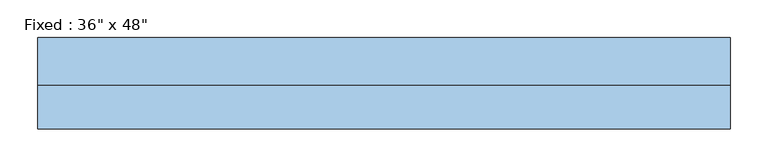
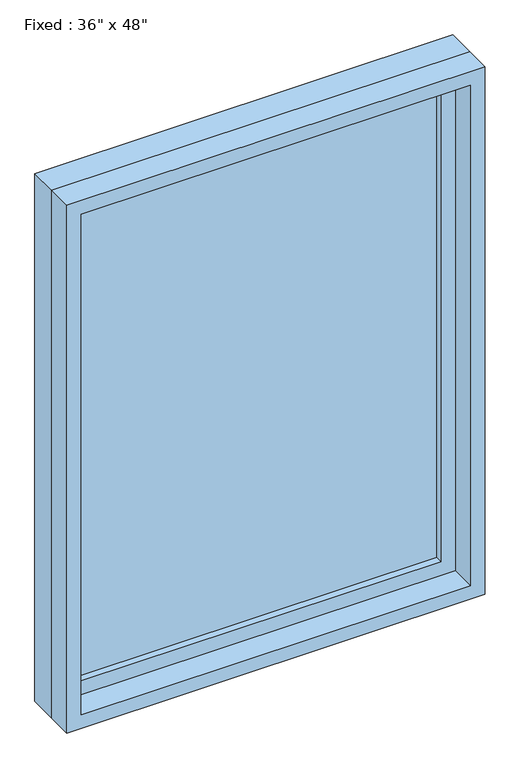
"""IFC4 building model written with IfcOpenShell, lengths in millimetres: window geometry."""

from ifc_helpers import new_model, si_unit, frame, origin, place, context, project, spatial, polyline, outline, extrude, source, transform, mapped, element, save


def window_51f22951(model_context):
    return source(origin(), model_context, "Body", "SweptSolid", [
        extrude(outline(polyline([(355.6, 12.7), (-431.8, 12.7), (-431.8, 25.4), (355.6, 25.4), (355.6, 12.7)])), frame((0.0, 0.0, 977.9), z_axis=(0.0, 0.0, 1.0), x_axis=(1.0, 0.0, 0.0)), (0.0, 0.0, 1.0), 1092.2),
        extrude(outline(polyline([(2114.55, -476.25), (933.45, -476.25), (933.45, 400.05), (2114.55, 400.05), (2114.55, -476.25)]), holes=[polyline([(2070.1, -431.8), (2070.1, 355.6), (977.9, 355.6), (977.9, -431.8), (2070.1, -431.8)])]), frame((0.0, -3.175, 0.0), z_axis=(0.0, 1.0, 0.0), x_axis=(0.0, 0.0, 1.0)), (0.0, 0.0, 1.0), 44.45),
        extrude(outline(polyline([(2133.6, -495.3), (914.4, -495.3), (914.4, 419.1), (2133.6, 419.1), (2133.6, -495.3)]), holes=[polyline([(2101.85, -463.55), (2101.85, 387.35), (946.15, 387.35), (946.15, -463.55), (2101.85, -463.55)])]), frame((0.0, -60.325, 0.0), z_axis=(0.0, 1.0, 0.0), x_axis=(0.0, 0.0, 1.0)), (0.0, 0.0, 1.0), 57.15),
        extrude(outline(polyline([(2133.6, 419.1), (2133.6, -495.3), (914.4, -495.3), (914.4, 419.1), (2133.6, 419.1)]), holes=[polyline([(2114.55, 400.05), (933.45, 400.05), (933.45, -476.25), (2114.55, -476.25), (2114.55, 400.05)])]), frame((0.0, -3.175, 0.0), z_axis=(0.0, 1.0, 0.0), x_axis=(0.0, 0.0, 1.0)), (0.0, 0.0, 1.0), 63.5),
    ])


if __name__ == "__main__":
    model = new_model("IFC4")
    model_context = context("Model", 3, world=origin())
    ifc_project = project(units=[si_unit("LENGTHUNIT", "METRE", prefix="MILLI")], contexts=[model_context])
    site = spatial("IfcSite", under=ifc_project)
    building = spatial("IfcBuilding", under=site)
    placement = place(None, origin())
    window_shape = window_51f22951(model_context)
    element("IfcWindow", 1, ObjectType="Fixed : 36\" x 48\"", at=placement, inside=building, context=model_context, shape_type="MappedRepresentation", body=[
        mapped(window_shape, transform((0.0, 0.0, 0.0), x_axis=(1.0, 0.0, 0.0), y_axis=(0.0, 1.0, 0.0), z_axis=(0.0, 0.0, 1.0))),
    ])
    save(model, "model.ifc")

# Revit data of these elements
# Type "Fixed : 36\" x 48\""
#   Type Mark = "10"
#   Construction Type Id = "GSP4R"
#   Assembly Code = "B2020100"
#   Analytic Construction = "1/8 in Pilkington single glazing"
#   Visual Light Transmittance = 0.9
#   Solar Heat Gain Coefficient = 0.78
#   Heat Transfer Coefficient (U) = 0.6496 BTU/(h·ft²·°F)
#   Height = 1219.2 mm
#   Default Sill Height = 914.4 mm
#   Width = 914.4 mm
#   Window Inset = 19.05 mm
#   Define Thermal Properties by = 1
#   Define Thermal Properties by = 1
#   Glass Pane Material = Glass
#   Sash Material = Sash
#   Wall Closure = (empty or 0)
# Element 1 (IfcWindow, "Fixed : 36\" x 48\"")
#   Materials on its faces: "Sash", "Glass"
# Materials
#   "Glass": class "Glass", colour RGB 154 182 205, transparency 0.5, Cost = 0
#   "Sash": class "Wood", colour RGB 224 178 126, transparency 0, Cost = 0
